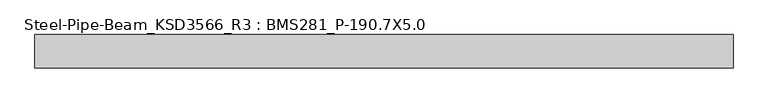
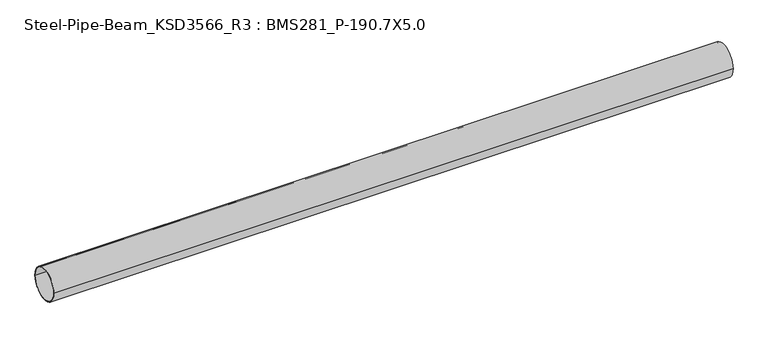
"""IFC4 building model written with IfcOpenShell, lengths in millimetres: member geometry, Steel-Pipe-Beam_KSD3566_R3 : BMS281_P-190.7X5.0."""

import ifcopenshell
import ifcopenshell.guid

model = None  # the IFC model being written
_history = None  # IfcOwnerHistory: only IFC2X3 demands one
_inside = {}  # id of a spatial element -> (the spatial element, [elements in it])
_under = {}  # id of a project, library or spatial element -> (it, [spatial elements below it])
_declared = {}  # id of a project -> (the project, [libraries it declares])
_typed = {}  # id of a type object -> (the type object, [elements of that type])
_made_of = {}  # id of a material, layer set ... -> (it, [elements and type objects made of it])


def new_model(schema):
    """Start an empty IFC model of exactly this schema.

    Asked for "IFC4X3", IfcOpenShell would pick the latest addendum, in which some entities
    have other attributes; the version numbers below select the first issue.
    IFC2X3 requires an IfcOwnerHistory on every rooted entity: one is made here for all.
    """
    global model, _history
    if schema == "IFC4X3":
        model = ifcopenshell.file(schema_version=(4, 3, 0, 0))
    else:
        model = ifcopenshell.file(schema=schema)
    _inside.clear()
    _under.clear()
    _declared.clear()
    _typed.clear()
    _made_of.clear()
    _history = None
    if model.schema == "IFC2X3":
        org = make("IfcOrganization", Name="unknown")
        user = make(
            "IfcPersonAndOrganization",
            ThePerson=make("IfcPerson", FamilyName="unknown"),
            TheOrganization=org,
        )
        app = make(
            "IfcApplication",
            ApplicationDeveloper=org,
            Version="unknown",
            ApplicationFullName="unknown",
            ApplicationIdentifier="unknown",
        )
        _history = make(
            "IfcOwnerHistory",
            OwningUser=user,
            OwningApplication=app,
            ChangeAction="ADDED",
            CreationDate=0,
        )
    return model


def make(cls, **values):
    """One entity of the class cls with the attributes given. An attribute that is None is left unset."""
    return model.create_entity(
        cls, **{name: value for name, value in values.items() if value is not None}
    )


def rooted(cls, **values):
    """An entity with a GlobalId (a new one), such as an element, a storey or a relation."""
    return make(cls, GlobalId=ifcopenshell.guid.new(), OwnerHistory=_history, **values)


def si_unit(unit_type, name, prefix=None):
    """IfcSIUnit, for example si_unit("LENGTHUNIT", "METRE", prefix="MILLI")."""
    return make("IfcSIUnit", UnitType=unit_type, Prefix=prefix, Name=name)


def assignment(units):
    """IfcUnitAssignment: the units of a project."""
    return None if units is None else make("IfcUnitAssignment", Units=units)


def point(xyz):
    """IfcCartesianPoint."""
    return None if xyz is None else make("IfcCartesianPoint", Coordinates=xyz)


def direction(xyz):
    """IfcDirection."""
    return None if xyz is None else make("IfcDirection", DirectionRatios=xyz)


def frame(location, z_axis=None, x_axis=None):
    """IfcAxis2Placement3D, a coordinate frame: its origin and axes. An axis left out is left unset."""
    return make(
        "IfcAxis2Placement3D",
        Location=point(location),
        Axis=direction(z_axis),
        RefDirection=direction(x_axis),
    )


def frame_2d(location, x_axis=None):
    """IfcAxis2Placement2D, a coordinate frame in the plane: its origin and x axis."""
    return make(
        "IfcAxis2Placement2D", Location=point(location), RefDirection=direction(x_axis)
    )


def origin():
    """The frame at (0, 0, 0) with its axes left unset."""
    return frame((0.0, 0.0, 0.0))


def origin_2d():
    """The frame at (0, 0) in the plane with its x axis left unset."""
    return frame_2d((0.0, 0.0))


def place(relative_to, where):
    """IfcLocalPlacement: puts the frame where relative to a parent placement (None: the world)."""
    return make(
        "IfcLocalPlacement", PlacementRelTo=relative_to, RelativePlacement=where
    )


def context(
    kind, dimensions, precision=None, world=None, true_north=None, identifier=None
):
    """IfcGeometricRepresentationContext, for example the 3D "Model" context."""
    return make(
        "IfcGeometricRepresentationContext",
        ContextIdentifier=identifier,
        ContextType=kind,
        CoordinateSpaceDimension=dimensions,
        Precision=precision,
        WorldCoordinateSystem=world,
        TrueNorth=true_north,
    )


def project(units=None, contexts=None):
    """IfcProject with its units and contexts."""
    return rooted(
        "IfcProject",
        Name="project",
        RepresentationContexts=contexts,
        UnitsInContext=assignment(units),
    )


def spatial(cls, under=None, at=None, **own):
    """A site, building, storey or space (cls), placed at a placement, below another one or the project."""
    s = rooted(cls, ObjectPlacement=at, **own)
    if under is not None:
        _under.setdefault(under.id(), (under, []))[1].append(s)
    return s


def circle_curve(where, radius):
    """IfcCircle in the frame where."""
    return make("IfcCircle", Position=where, Radius=radius)


def trimmed(basis, trim1, trim2, sense, master):
    """IfcTrimmedCurve: the piece of a basis curve between two trims."""
    return make(
        "IfcTrimmedCurve",
        BasisCurve=basis,
        Trim1=trim1,
        Trim2=trim2,
        SenseAgreement=sense,
        MasterRepresentation=master,
    )


def segment(curve, same_sense, transition):
    """IfcCompositeCurveSegment."""
    return make(
        "IfcCompositeCurveSegment",
        Transition=transition,
        SameSense=same_sense,
        ParentCurve=curve,
    )


def composite_curve(segments, self_intersect=None):
    """IfcCompositeCurve: segments joined end to end."""
    return make("IfcCompositeCurve", Segments=segments, SelfIntersect=self_intersect)


def outline(outer, holes=None, kind="AREA"):
    """IfcArbitraryClosedProfileDef: a profile drawn as a closed curve; with holes, ...WithVoids."""
    if holes is None:
        return make("IfcArbitraryClosedProfileDef", ProfileType=kind, OuterCurve=outer)
    return make(
        "IfcArbitraryProfileDefWithVoids",
        ProfileType=kind,
        OuterCurve=outer,
        InnerCurves=holes,
    )


def extrude(swept, where, along, depth):
    """IfcExtrudedAreaSolid: the profile swept, set in the frame where, extruded along a direction by depth."""
    return make(
        "IfcExtrudedAreaSolid",
        SweptArea=swept,
        Position=where,
        ExtrudedDirection=direction(along),
        Depth=depth,
    )


def shape(context_of_items, identifier, shape_type, items):
    """IfcShapeRepresentation: the items that make up one representation, for example the "Body"."""
    return make(
        "IfcShapeRepresentation",
        ContextOfItems=context_of_items,
        RepresentationIdentifier=identifier,
        RepresentationType=shape_type,
        Items=items,
    )


def source(mapping_origin, context_of_items, identifier, shape_type, items):
    """IfcRepresentationMap: a shape defined once, which mapped items show again and again."""
    return make(
        "IfcRepresentationMap",
        MappingOrigin=mapping_origin,
        MappedRepresentation=shape(context_of_items, identifier, shape_type, items),
    )


def transform(
    local_origin,
    x_axis=None,
    y_axis=None,
    z_axis=None,
    scale=None,
    scale2=None,
    scale3=None,
    uniform=True,
):
    """IfcCartesianTransformationOperator3D, or its non-uniform kind. x_axis, y_axis, z_axis: its Axis1, 2, 3."""
    if uniform:
        return make(
            "IfcCartesianTransformationOperator3D",
            Axis1=direction(x_axis),
            Axis2=direction(y_axis),
            LocalOrigin=point(local_origin),
            Scale=scale,
            Axis3=direction(z_axis),
        )
    return make(
        "IfcCartesianTransformationOperator3DnonUniform",
        Axis1=direction(x_axis),
        Axis2=direction(y_axis),
        LocalOrigin=point(local_origin),
        Scale=scale,
        Axis3=direction(z_axis),
        Scale2=scale2,
        Scale3=scale3,
    )


def mapped(mapping_source, mapping_target):
    """IfcMappedItem: shows the shape of a source again, moved by a transform."""
    return make(
        "IfcMappedItem", MappingSource=mapping_source, MappingTarget=mapping_target
    )


def made_of(thing, what):
    """Note that an element or type object is made of a material, layer set ...; save() writes the relation."""
    if what is not None:
        _made_of.setdefault(what.id(), (what, []))[1].append(thing)
    return thing


def element(
    cls,
    number,
    at=None,
    inside=None,
    cuts=None,
    type_object=None,
    material=None,
    context=None,
    identifier="Body",
    shape_type=None,
    held_by="IfcProductDefinitionShape",
    body=None,
    shapes=None,
    **own,
):
    """One element of the class cls, such as IfcWall. Its Tag is "e" and its number.

    at: its placement. inside: the storey or other place that contains it. cuts: it is an
    opening in that element (IfcRelVoidsElement). A single representation is given by context,
    identifier, shape_type and body (its items); several are given by shapes. held_by: the class
    of the entity that holds the representations. save() writes the other relations.
    """
    e = rooted(cls, Tag="e%d" % number, ObjectPlacement=at, **own)
    if body is not None:
        shapes = [shape(context, identifier, shape_type, body)]
    if shapes is not None:
        e.Representation = make(held_by, Representations=shapes)
    if inside is not None:
        _inside.setdefault(inside.id(), (inside, []))[1].append(e)
    if cuts is not None:
        rooted(
            "IfcRelVoidsElement", RelatingBuildingElement=cuts, RelatedOpeningElement=e
        )
    if type_object is not None:
        _typed.setdefault(type_object.id(), (type_object, []))[1].append(e)
    return made_of(e, material)


def aggregate(whole, parts):
    """IfcRelAggregates: a whole, such as a stair, and the parts it consists of."""
    return rooted("IfcRelAggregates", RelatingObject=whole, RelatedObjects=parts)


def save(model, path):
    """Write the relations noted so far, then the file.

    IfcRelAggregates (storeys below a building ...), IfcRelContainedInSpatialStructure (elements
    in a storey), IfcRelDefinesByType, IfcRelAssociatesMaterial and IfcRelDeclares: one each for
    every whole, place, type object, material and project.
    """
    for whole, parts in _under.values():
        aggregate(whole, parts)
    for where, things in _inside.values():
        rooted(
            "IfcRelContainedInSpatialStructure",
            RelatedElements=things,
            RelatingStructure=where,
        )
    for kind, things in _typed.values():
        rooted("IfcRelDefinesByType", RelatedObjects=things, RelatingType=kind)
    for what, things in _made_of.values():
        rooted("IfcRelAssociatesMaterial", RelatedObjects=things, RelatingMaterial=what)
    for by, libraries in _declared.values():
        rooted("IfcRelDeclares", RelatingContext=by, RelatedDefinitions=libraries)
    model.write(path)


def steel_pipe_beam_ksd3566_r3_bms281_p_190_7x5_0_fa8c165e(model_context):
    return source(origin(), model_context, "Body", "SweptSolid", [
        extrude(outline(composite_curve([segment(trimmed(circle_curve(origin_2d(), 95.35), [point((-95.35, 0.0))], [point((95.35, 0.0))], False, "CARTESIAN"), True, "CONTINUOUS"), segment(trimmed(circle_curve(origin_2d(), 95.35), [point((95.35, 0.0))], [point((-95.35, 0.0))], False, "CARTESIAN"), True, "CONTINUOUS")], self_intersect=False), holes=[composite_curve([segment(trimmed(circle_curve(origin_2d(), 90.35), [point((90.35, 0.0))], [point((-90.35, 0.0))], True, "CARTESIAN"), True, "CONTINUOUS"), segment(trimmed(circle_curve(origin_2d(), 90.35), [point((-90.35, 0.0))], [point((90.35, 0.0))], True, "CARTESIAN"), True, "CONTINUOUS")], self_intersect=False)]), frame((-2003.1065044, 0.0, 0.0), z_axis=(1.0, 0.0, 0.0), x_axis=(0.0, 1.0, 0.0)), (0.0, 0.0, 1.0), 3968.5849078),
    ])


if __name__ == "__main__":
    model = new_model("IFC4")
    model_context = context("Model", 3, world=origin())
    ifc_project = project(units=[si_unit("LENGTHUNIT", "METRE", prefix="MILLI")], contexts=[model_context])
    site = spatial("IfcSite", under=ifc_project)
    building = spatial("IfcBuilding", under=site)
    placement = place(None, origin())
    steel_pipe_beam_ksd3566_r3_bms281_p_190_7x5_0_shape = steel_pipe_beam_ksd3566_r3_bms281_p_190_7x5_0_fa8c165e(model_context)
    element("IfcMember", 1, ObjectType="Steel-Pipe-Beam_KSD3566_R3 : BMS281_P-190.7X5.0", at=placement, inside=building, context=model_context, shape_type="MappedRepresentation", body=[
        mapped(steel_pipe_beam_ksd3566_r3_bms281_p_190_7x5_0_shape, transform((0.0, 0.0, 0.0), x_axis=(1.0, 0.0, 0.0), y_axis=(0.0, 1.0, 0.0), z_axis=(0.0, 0.0, 1.0))),
    ])
    save(model, "model.ifc")

# Revit data of these elements
# Type "Steel-Pipe-Beam_KSD3566_R3 : BMS281_P-190.7X5.0"
#   Keynote = "P-190.7X5.0"
#   SteelWeight = "Light"
#   t = 0.0050 m
#   Surface Area = 0.599102 m²/m
#   Section Area = 29.1697 cm²
#   Mass per Unit Length = 22.8982 kg/m
#   Length [instance default] = 1.5000 m
#   D = 0.1907 m
#   hec_material4 [instance default] = none
#   hec_material3 [instance default] = none
#   hec_material2 [instance default] = none
#   hec_material1 [instance default] = none
#   Structural Material [instance default] = Steel, 45-345
#   Assembly Code = ""
# Element 1 (IfcMember, "Steel-Pipe-Beam_KSD3566_R3 : BMS281_P-190.7X5.0")
#   Structural Material = none
# Materials
#   "Steel, 45-345": class "Metal", colour RGB 189 187 185, transparency 0, Description = "Steel 345 MPa", Cost = 0
